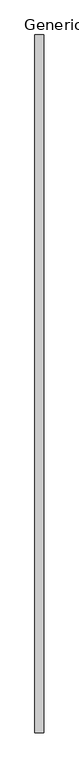
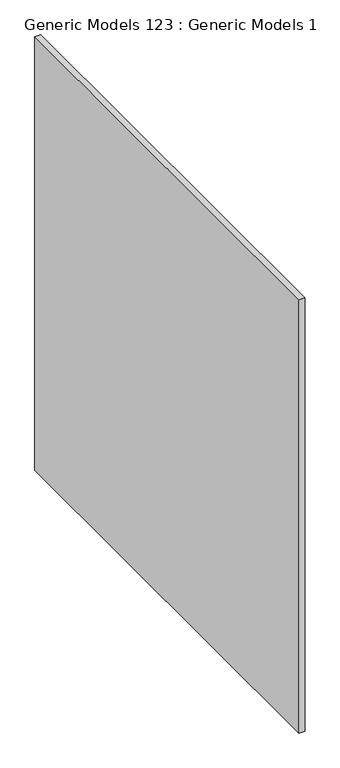
"""IFC4 building model written with IfcOpenShell, lengths in millimetres: proxy geometry, Generic Models 123 : Generic Models 1."""

from ifc_helpers import new_model, si_unit, frame, origin, place, context, project, spatial, polyline, outline, extrude, source, transform, mapped, element, save


def generic_models_123_generic_models_1_1fe7ed5f(model_context):
    return source(origin(), model_context, "Body", "SweptSolid", [
        extrude(outline(polyline([(46827.9235531, 1219.2), (46843.7985531, 1219.2), (46843.7985531, 0.0), (46827.9235531, 0.0), (46827.9235531, 1219.2)])), frame((0.0, 0.0, -219.626067), z_axis=(0.0, 0.0, 1.0), x_axis=(1.0, 0.0, 0.0)), (0.0, 0.0, 1.0), 1219.2),
    ])


if __name__ == "__main__":
    model = new_model("IFC4")
    model_context = context("Model", 3, world=origin())
    ifc_project = project(units=[si_unit("LENGTHUNIT", "METRE", prefix="MILLI")], contexts=[model_context])
    site = spatial("IfcSite", under=ifc_project)
    building = spatial("IfcBuilding", under=site)
    placement = place(None, origin())
    generic_models_123_generic_models_1_shape = generic_models_123_generic_models_1_1fe7ed5f(model_context)
    element("IfcBuildingElementProxy", 1, Name="Generic Models 123 : Generic Models 1", ObjectType="Generic Models 123 : Generic Models 1", at=placement, inside=building, context=model_context, shape_type="MappedRepresentation", body=[
        mapped(generic_models_123_generic_models_1_shape, transform((0.0, 0.0, 0.0), x_axis=(1.0, 0.0, 0.0), y_axis=(0.0, 1.0, 0.0), z_axis=(0.0, 0.0, 1.0))),
    ])
    save(model, "model.ifc")

# Revit data of these elements
# Element 1 (IfcBuildingElementProxy, "Generic Models 123 : Generic Models 1")
#   Materials on its faces: "5/8\" GYP. BD"
# Materials
#   "5/8\" GYP. BD": class "Generic", colour RGB 255 255 255, transparency 0, Description = "Gypsum Wall Board", Cost = 0
